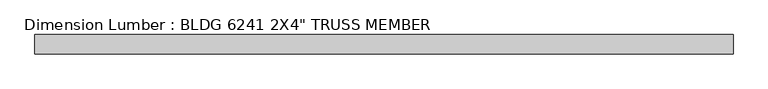
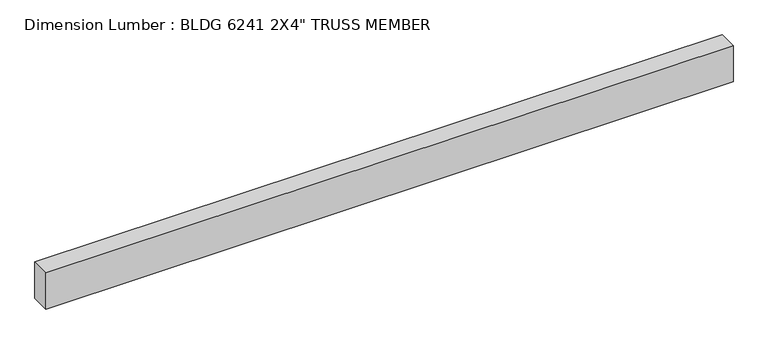
"""IFC4 building model written with IfcOpenShell, lengths in millimetres: beam geometry."""

from ifc_helpers import new_model, si_unit, frame, origin, place, context, project, spatial, polyline, outline, extrude, source, transform, mapped, element, save


def beam_dc030418(model_context):
    return source(origin(), model_context, "Body", "SweptSolid", [
        extrude(outline(polyline([(914.4, 25.4), (914.4, -25.4), (-914.4, -25.4), (-914.4, 25.4), (914.4, 25.4)])), frame((0.0, 0.0, -50.8), z_axis=(0.0, 0.0, 1.0), x_axis=(1.0, 0.0, 0.0)), (0.0, 0.0, 1.0), 101.6),
    ])


if __name__ == "__main__":
    model = new_model("IFC4")
    model_context = context("Model", 3, world=origin())
    ifc_project = project(units=[si_unit("LENGTHUNIT", "METRE", prefix="MILLI")], contexts=[model_context])
    site = spatial("IfcSite", under=ifc_project)
    building = spatial("IfcBuilding", under=site)
    placement = place(None, origin())
    beam_shape = beam_dc030418(model_context)
    element("IfcBeam", 1, ObjectType="Dimension Lumber : BLDG 6241 2X4\" TRUSS MEMBER", at=placement, inside=building, context=model_context, shape_type="MappedRepresentation", body=[
        mapped(beam_shape, transform((0.0, 0.0, 0.0), x_axis=(1.0, 0.0, 0.0), y_axis=(0.0, 1.0, 0.0), z_axis=(0.0, 0.0, 1.0))),
    ])
    save(model, "model.ifc")

# Revit data of these elements
# Type "Dimension Lumber : BLDG 6241 2X4\" TRUSS MEMBER"
#   Assembly Code = "B10"
#   A = 0.273472 SF
#   Length [instance default] = 5' - 0"
#   b = 0' - 2"
#   d = 0' - 4"
#   Structural Material [instance default] = Softwood, Lumber
# Element 1 (IfcBeam, "Dimension Lumber : BLDG 6241 2X4\" TRUSS MEMBER")
#   Materials on its faces: "Softwood, Lumber"
# Materials
#   "Softwood, Lumber": class "Wood", colour RGB 223 192 134, transparency 0, Description = "Pinus Echinata", Cost = 0
